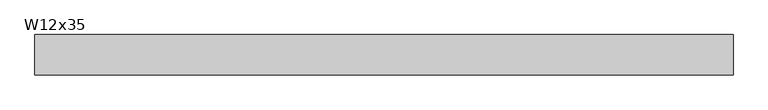
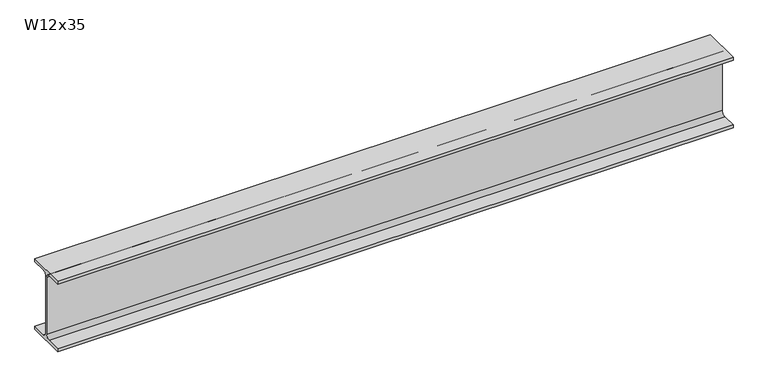
"""IFC4 building model written with IfcOpenShell, lengths in millimetres: beam geometry, RME W-Wide Flange : W12x35."""

from ifc_helpers import new_model, si_unit, point, frame, frame_2d, origin, place, context, project, spatial, polyline, circle_curve, trimmed, segment, composite_curve, outline, extrude, source, transform, mapped, element, save


def w12x35_e1547693(model_context):
    return source(origin(), model_context, "Body", "SweptSolid", [
        extrude(outline(composite_curve([segment(polyline([(83.312, -145.542), (83.312, -158.75), (-83.312, -158.75), (-83.312, -145.542), (-20.7645, -145.542)]), True, "CONTINUOUS"), segment(trimmed(circle_curve(frame_2d((-20.7645, -128.5875)), 16.9545), [point((-20.7645, -145.542))], [point((-3.81, -128.5875))], True, "CARTESIAN"), True, "CONTINUOUS"), segment(polyline([(-3.81, -128.5875), (-3.81, 128.5875)]), True, "CONTINUOUS"), segment(trimmed(circle_curve(frame_2d((-20.7645, 128.5875)), 16.9545), [point((-3.81, 128.5875))], [point((-20.7645, 145.542))], True, "CARTESIAN"), True, "CONTINUOUS"), segment(polyline([(-20.7645, 145.542), (-83.312, 145.542), (-83.312, 158.75), (83.312, 158.75), (83.312, 145.542), (20.7645, 145.542)]), True, "CONTINUOUS"), segment(trimmed(circle_curve(frame_2d((20.7645, 128.5875)), 16.9545), [point((20.7645, 145.542))], [point((3.81, 128.5875))], True, "CARTESIAN"), True, "CONTINUOUS"), segment(polyline([(3.81, 128.5875), (3.81, -128.5875)]), True, "CONTINUOUS"), segment(trimmed(circle_curve(frame_2d((20.7645, -128.5875)), 16.9545), [point((3.81, -128.5875))], [point((20.7645, -145.542))], True, "CARTESIAN"), True, "CONTINUOUS"), segment(polyline([(20.7645, -145.542), (83.312, -145.542)]), True, "CONTINUOUS")], self_intersect=False)), frame((-1441.210987, 0.0, 0.0), z_axis=(1.0, 0.0, 0.0), x_axis=(0.0, 1.0, 0.0)), (0.0, 0.0, 1.0), 2875.7320431),
    ])


if __name__ == "__main__":
    model = new_model("IFC4")
    model_context = context("Model", 3, world=origin())
    ifc_project = project(units=[si_unit("LENGTHUNIT", "METRE", prefix="MILLI")], contexts=[model_context])
    site = spatial("IfcSite", under=ifc_project)
    building = spatial("IfcBuilding", under=site)
    placement = place(None, origin())
    w12x35_shape = w12x35_e1547693(model_context)
    element("IfcBeam", 1, ObjectType="RME W-Wide Flange : W12x35", at=placement, inside=building, context=model_context, shape_type="MappedRepresentation", body=[
        mapped(w12x35_shape, transform((0.0, 0.0, 0.0), x_axis=(1.0, 0.0, 0.0), y_axis=(0.0, 1.0, 0.0), z_axis=(0.0, 0.0, 1.0))),
    ])
    save(model, "model.ifc")

# Revit data of these elements
# Type "RME W-Wide Flange : W12x35"
#   WELD P [instance default] = ""
#   WELD LE [instance default] = ""
#   WELD D [instance default] = ""
#   TOP SECTION SIZE [instance default] = ""
#   TOP SECTION LENGTH [instance default] = ""
#   REMARKS [instance default] = ""
#   REINF TYPE [instance default] = ""
#   Nominal Size = "W24"
#   End Bearing Capacity [instance default] = ""
#   BOT SECTION SIZE [instance default] = ""
#   BOT SECTION LENGTH [instance default] = ""
#   Assembly Code = "B10"
#   W = 35
#   Start Extension Calculation [instance default] = 10' - 0"
#   Start Extension [instance default] = -0' - 0 1/2"
#   End Extension Calculation [instance default] = 10' - 0"
#   End Extension [instance default] = -0' - 0 1/2"
#   Length [instance default] = 5' - 0"
#   bf = 0' - 6.56"
#   d = 1' - 0 1/2"
#   k = 0' - 1 3/16"
#   k2 = 0' - 0.6675"
#   tf = 0' - 0.52"
#   tw = 0' - 0.3"
#   A = 0.0715278 SF
#   Structural Material [instance default] = Metal - Steel - ASTM A992
# Element 1 (IfcBeam, "RME W-Wide Flange : W12x35")
#   Length = 10' - 1.02542"
#   Materials on its faces: "Metal - Steel - ASTM A992"
# Materials
#   "Metal - Steel - ASTM A992": class "Metal", colour RGB 255 128 0, transparency 0
